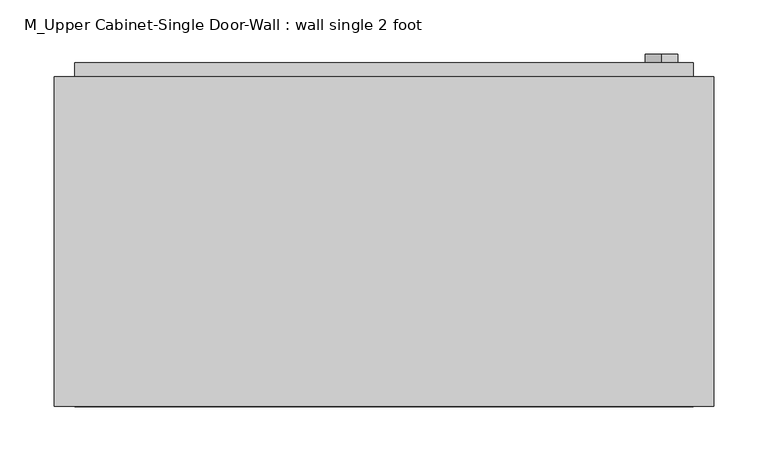
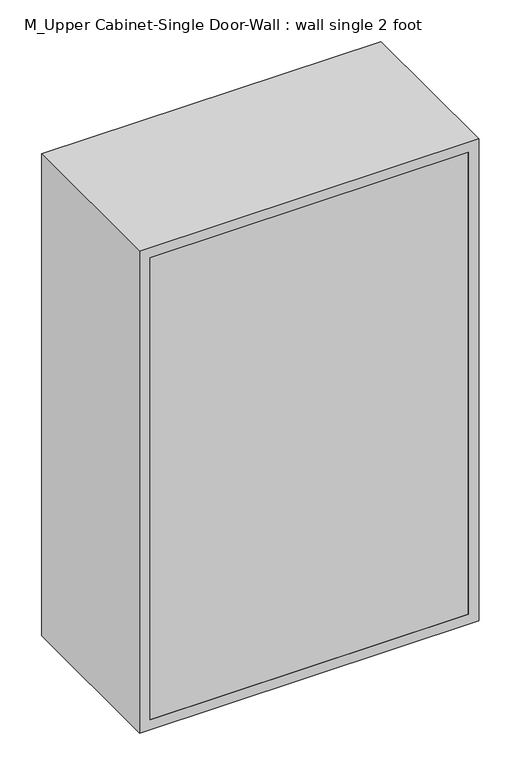
"""IFC4 building model written with IfcOpenShell, lengths in millimetres: furniture geometry, M_Upper Cabinet-Single Door-Wall : wall single 2 foot."""

from ifc_helpers import new_model, si_unit, point, frame, frame_2d, origin, place, context, project, spatial, polyline, circle_curve, trimmed, segment, composite_curve, outline, extrude, source, transform, mapped, element, save


def m_upper_cabinet_single_door_wall_wall_single_2_foot_bbc4a682(model_context):
    return source(origin(), model_context, "Body", "SweptSolid", [
        extrude(outline(polyline([(-255.9788372, 373.85625), (315.5211628, 373.85625), (315.5211628, 342.10625), (-255.9788372, 342.10625), (-255.9788372, 373.85625)])), frame((0.0, 0.0, 1104.65), z_axis=(0.0, 0.0, 1.0), x_axis=(1.0, 0.0, 0.0)), (0.0, 0.0, 1.0), 876.3),
        extrude(outline(polyline([(315.5211628, 56.35625), (-255.9788372, 56.35625), (-255.9788372, 75.40625), (315.5211628, 75.40625), (315.5211628, 56.35625)])), frame((0.0, 0.0, 1104.65), z_axis=(0.0, 0.0, 1.0), x_axis=(1.0, 0.0, 0.0)), (0.0, 0.0, 1.0), 876.3),
        extrude(outline(polyline([(2000.0, -275.0288372), (1085.6, -275.0288372), (1085.6, 334.5711628), (2000.0, 334.5711628), (2000.0, -275.0288372)]), holes=[polyline([(1980.95, -255.9788372), (1980.95, 315.5211628), (1104.65, 315.5211628), (1104.65, -255.9788372), (1980.95, -255.9788372)])]), frame((0.0, 56.35625, 0.0), z_axis=(0.0, 1.0, 0.0), x_axis=(0.0, 0.0, 1.0)), (0.0, 0.0, 1.0), 304.8),
        extrude(outline(composite_curve([segment(trimmed(circle_curve(frame_2d((1280.6953371, 285.9613252)), 15.0), [point((1265.6953371, 285.9613252))], [point((1295.6953371, 285.9613252))], False, "CARTESIAN"), True, "CONTINUOUS"), segment(trimmed(circle_curve(frame_2d((1280.6953371, 285.9613252)), 15.0), [point((1295.6953371, 285.9613252))], [point((1265.6953371, 285.9613252))], False, "CARTESIAN"), True, "CONTINUOUS")], self_intersect=False)), frame((0.0, 373.85625, 0.0), z_axis=(0.0, 1.0, 0.0), x_axis=(0.0, 0.0, 1.0)), (0.0, 0.0, 1.0), 8.0),
    ])


if __name__ == "__main__":
    model = new_model("IFC4")
    model_context = context("Model", 3, world=origin())
    ifc_project = project(units=[si_unit("LENGTHUNIT", "METRE", prefix="MILLI")], contexts=[model_context])
    site = spatial("IfcSite", under=ifc_project)
    building = spatial("IfcBuilding", under=site)
    placement = place(None, origin())
    m_upper_cabinet_single_door_wall_wall_single_2_foot_shape = m_upper_cabinet_single_door_wall_wall_single_2_foot_bbc4a682(model_context)
    element("IfcFurniture", 1, ObjectType="M_Upper Cabinet-Single Door-Wall : wall single 2 foot", at=placement, inside=building, context=model_context, shape_type="MappedRepresentation", body=[
        mapped(m_upper_cabinet_single_door_wall_wall_single_2_foot_shape, transform((0.0, 0.0, 0.0), x_axis=(1.0, 0.0, 0.0), y_axis=(0.0, 1.0, 0.0), z_axis=(0.0, 0.0, 1.0))),
    ])
    save(model, "model.ifc")

# Revit data of these elements
# Type "M_Upper Cabinet-Single Door-Wall : wall single 2 foot"
#   Depth = 1' - 0"
#   Height = 3' - 0"
#   Top Of Cabinet = 6' - 6.74016"
#   Width = 2' - 0"
#   Cabinet Material = Base cabinet 2120100 Aspekt - 83012120100 - White
#   Door/Drawer Material = Base cabinet 2120100 Aspekt - 83012120100 - White
#   Handle Material = Cabinets - Handles
#   Default Elevation = 0
# Element 1 (IfcFurniture, "M_Upper Cabinet-Single Door-Wall : wall single 2 foot")
#   Materials on its faces: "Base cabinet 2120100 Aspekt - 83012120100 - White"
# Materials
#   "Base cabinet 2120100 Aspekt - 83012120100 - White": class "Miscellaneous", colour RGB 255 255 255, transparency 0, Manufacturer = "Marbodal", URL = "http://www.marbodal.se", Cost = 0
#   "Cabinets - Handles": class "Metal", colour RGB 57 57 57, transparency 0
